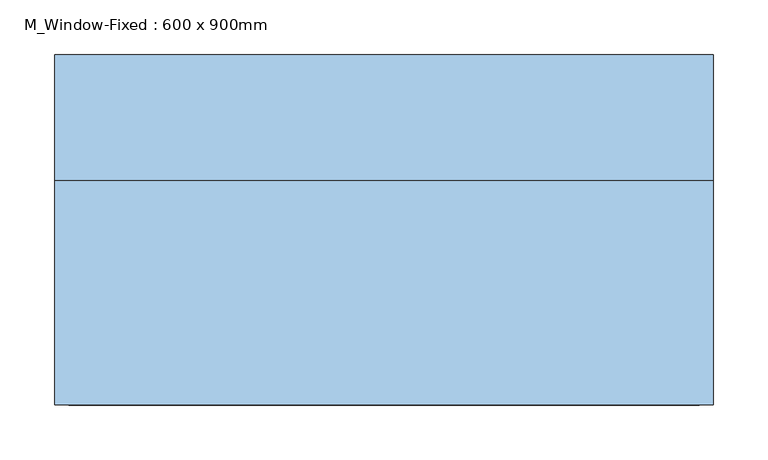
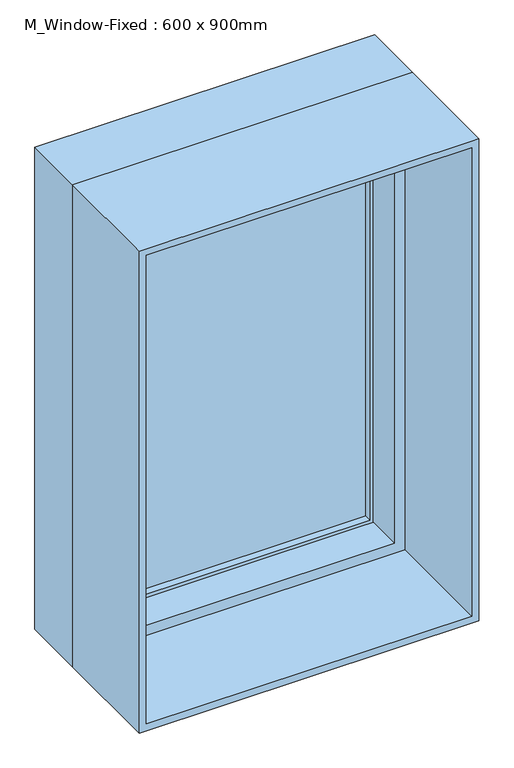
"""IFC4 building model written with IfcOpenShell, lengths in millimetres: window geometry, M_Window-Fixed : 600 x 900mm."""

import ifcopenshell
import ifcopenshell.guid

model = None  # the IFC model being written
_history = None  # IfcOwnerHistory: only IFC2X3 demands one
_inside = {}  # id of a spatial element -> (the spatial element, [elements in it])
_under = {}  # id of a project, library or spatial element -> (it, [spatial elements below it])
_declared = {}  # id of a project -> (the project, [libraries it declares])
_typed = {}  # id of a type object -> (the type object, [elements of that type])
_made_of = {}  # id of a material, layer set ... -> (it, [elements and type objects made of it])


def new_model(schema):
    """Start an empty IFC model of exactly this schema.

    Asked for "IFC4X3", IfcOpenShell would pick the latest addendum, in which some entities
    have other attributes; the version numbers below select the first issue.
    IFC2X3 requires an IfcOwnerHistory on every rooted entity: one is made here for all.
    """
    global model, _history
    if schema == "IFC4X3":
        model = ifcopenshell.file(schema_version=(4, 3, 0, 0))
    else:
        model = ifcopenshell.file(schema=schema)
    _inside.clear()
    _under.clear()
    _declared.clear()
    _typed.clear()
    _made_of.clear()
    _history = None
    if model.schema == "IFC2X3":
        org = make("IfcOrganization", Name="unknown")
        user = make(
            "IfcPersonAndOrganization",
            ThePerson=make("IfcPerson", FamilyName="unknown"),
            TheOrganization=org,
        )
        app = make(
            "IfcApplication",
            ApplicationDeveloper=org,
            Version="unknown",
            ApplicationFullName="unknown",
            ApplicationIdentifier="unknown",
        )
        _history = make(
            "IfcOwnerHistory",
            OwningUser=user,
            OwningApplication=app,
            ChangeAction="ADDED",
            CreationDate=0,
        )
    return model


def make(cls, **values):
    """One entity of the class cls with the attributes given. An attribute that is None is left unset."""
    return model.create_entity(
        cls, **{name: value for name, value in values.items() if value is not None}
    )


def rooted(cls, **values):
    """An entity with a GlobalId (a new one), such as an element, a storey or a relation."""
    return make(cls, GlobalId=ifcopenshell.guid.new(), OwnerHistory=_history, **values)


def si_unit(unit_type, name, prefix=None):
    """IfcSIUnit, for example si_unit("LENGTHUNIT", "METRE", prefix="MILLI")."""
    return make("IfcSIUnit", UnitType=unit_type, Prefix=prefix, Name=name)


def assignment(units):
    """IfcUnitAssignment: the units of a project."""
    return None if units is None else make("IfcUnitAssignment", Units=units)


def point(xyz):
    """IfcCartesianPoint."""
    return None if xyz is None else make("IfcCartesianPoint", Coordinates=xyz)


def direction(xyz):
    """IfcDirection."""
    return None if xyz is None else make("IfcDirection", DirectionRatios=xyz)


def frame(location, z_axis=None, x_axis=None):
    """IfcAxis2Placement3D, a coordinate frame: its origin and axes. An axis left out is left unset."""
    return make(
        "IfcAxis2Placement3D",
        Location=point(location),
        Axis=direction(z_axis),
        RefDirection=direction(x_axis),
    )


def origin():
    """The frame at (0, 0, 0) with its axes left unset."""
    return frame((0.0, 0.0, 0.0))


def place(relative_to, where):
    """IfcLocalPlacement: puts the frame where relative to a parent placement (None: the world)."""
    return make(
        "IfcLocalPlacement", PlacementRelTo=relative_to, RelativePlacement=where
    )


def context(
    kind, dimensions, precision=None, world=None, true_north=None, identifier=None
):
    """IfcGeometricRepresentationContext, for example the 3D "Model" context."""
    return make(
        "IfcGeometricRepresentationContext",
        ContextIdentifier=identifier,
        ContextType=kind,
        CoordinateSpaceDimension=dimensions,
        Precision=precision,
        WorldCoordinateSystem=world,
        TrueNorth=true_north,
    )


def project(units=None, contexts=None):
    """IfcProject with its units and contexts."""
    return rooted(
        "IfcProject",
        Name="project",
        RepresentationContexts=contexts,
        UnitsInContext=assignment(units),
    )


def spatial(cls, under=None, at=None, **own):
    """A site, building, storey or space (cls), placed at a placement, below another one or the project."""
    s = rooted(cls, ObjectPlacement=at, **own)
    if under is not None:
        _under.setdefault(under.id(), (under, []))[1].append(s)
    return s


def polyline(points):
    """IfcPolyline through the points."""
    return make("IfcPolyline", Points=[point(p) for p in points])


def outline(outer, holes=None, kind="AREA"):
    """IfcArbitraryClosedProfileDef: a profile drawn as a closed curve; with holes, ...WithVoids."""
    if holes is None:
        return make("IfcArbitraryClosedProfileDef", ProfileType=kind, OuterCurve=outer)
    return make(
        "IfcArbitraryProfileDefWithVoids",
        ProfileType=kind,
        OuterCurve=outer,
        InnerCurves=holes,
    )


def extrude(swept, where, along, depth):
    """IfcExtrudedAreaSolid: the profile swept, set in the frame where, extruded along a direction by depth."""
    return make(
        "IfcExtrudedAreaSolid",
        SweptArea=swept,
        Position=where,
        ExtrudedDirection=direction(along),
        Depth=depth,
    )


def faces_of(points, faces, orient=None, outer=None):
    """IfcFace entities. A face is a list of loops; a loop is a list of indices into points, from 0.

    orient and outer hold one flag for each loop. By default every Orientation is true, the
    first loop of a face is its IfcFaceOuterBound and the others are IfcFaceBound.
    """
    made = []
    for i, loops in enumerate(faces):
        bounds = []
        for j, loop in enumerate(loops):
            is_outer = j == 0 if outer is None else outer[i][j]
            bounds.append(
                make(
                    "IfcFaceOuterBound" if is_outer else "IfcFaceBound",
                    Bound=make("IfcPolyLoop", Polygon=[points[k] for k in loop]),
                    Orientation=True if orient is None else orient[i][j],
                )
            )
        made.append(make("IfcFace", Bounds=bounds))
    return made


def faceted_brep(points, faces, orient=None, outer=None, voids=None):
    """IfcFacetedBrep: a solid bounded by flat faces; with voids (closed shells), ...WithVoids."""
    shared = [point(p) for p in points]
    hull = make("IfcClosedShell", CfsFaces=faces_of(shared, faces, orient, outer))
    if voids is None:
        return make("IfcFacetedBrep", Outer=hull)
    return make(
        "IfcFacetedBrepWithVoids",
        Outer=hull,
        Voids=[
            make(cls, CfsFaces=faces_of(shared, fs, o, b)) for cls, fs, o, b in voids
        ],
    )


def shape(context_of_items, identifier, shape_type, items):
    """IfcShapeRepresentation: the items that make up one representation, for example the "Body"."""
    return make(
        "IfcShapeRepresentation",
        ContextOfItems=context_of_items,
        RepresentationIdentifier=identifier,
        RepresentationType=shape_type,
        Items=items,
    )


def source(mapping_origin, context_of_items, identifier, shape_type, items):
    """IfcRepresentationMap: a shape defined once, which mapped items show again and again."""
    return make(
        "IfcRepresentationMap",
        MappingOrigin=mapping_origin,
        MappedRepresentation=shape(context_of_items, identifier, shape_type, items),
    )


def transform(
    local_origin,
    x_axis=None,
    y_axis=None,
    z_axis=None,
    scale=None,
    scale2=None,
    scale3=None,
    uniform=True,
):
    """IfcCartesianTransformationOperator3D, or its non-uniform kind. x_axis, y_axis, z_axis: its Axis1, 2, 3."""
    if uniform:
        return make(
            "IfcCartesianTransformationOperator3D",
            Axis1=direction(x_axis),
            Axis2=direction(y_axis),
            LocalOrigin=point(local_origin),
            Scale=scale,
            Axis3=direction(z_axis),
        )
    return make(
        "IfcCartesianTransformationOperator3DnonUniform",
        Axis1=direction(x_axis),
        Axis2=direction(y_axis),
        LocalOrigin=point(local_origin),
        Scale=scale,
        Axis3=direction(z_axis),
        Scale2=scale2,
        Scale3=scale3,
    )


def mapped(mapping_source, mapping_target):
    """IfcMappedItem: shows the shape of a source again, moved by a transform."""
    return make(
        "IfcMappedItem", MappingSource=mapping_source, MappingTarget=mapping_target
    )


def made_of(thing, what):
    """Note that an element or type object is made of a material, layer set ...; save() writes the relation."""
    if what is not None:
        _made_of.setdefault(what.id(), (what, []))[1].append(thing)
    return thing


def element(
    cls,
    number,
    at=None,
    inside=None,
    cuts=None,
    type_object=None,
    material=None,
    context=None,
    identifier="Body",
    shape_type=None,
    held_by="IfcProductDefinitionShape",
    body=None,
    shapes=None,
    **own,
):
    """One element of the class cls, such as IfcWall. Its Tag is "e" and its number.

    at: its placement. inside: the storey or other place that contains it. cuts: it is an
    opening in that element (IfcRelVoidsElement). A single representation is given by context,
    identifier, shape_type and body (its items); several are given by shapes. held_by: the class
    of the entity that holds the representations. save() writes the other relations.
    """
    e = rooted(cls, Tag="e%d" % number, ObjectPlacement=at, **own)
    if body is not None:
        shapes = [shape(context, identifier, shape_type, body)]
    if shapes is not None:
        e.Representation = make(held_by, Representations=shapes)
    if inside is not None:
        _inside.setdefault(inside.id(), (inside, []))[1].append(e)
    if cuts is not None:
        rooted(
            "IfcRelVoidsElement", RelatingBuildingElement=cuts, RelatedOpeningElement=e
        )
    if type_object is not None:
        _typed.setdefault(type_object.id(), (type_object, []))[1].append(e)
    return made_of(e, material)


def aggregate(whole, parts):
    """IfcRelAggregates: a whole, such as a stair, and the parts it consists of."""
    return rooted("IfcRelAggregates", RelatingObject=whole, RelatedObjects=parts)


def save(model, path):
    """Write the relations noted so far, then the file.

    IfcRelAggregates (storeys below a building ...), IfcRelContainedInSpatialStructure (elements
    in a storey), IfcRelDefinesByType, IfcRelAssociatesMaterial and IfcRelDeclares: one each for
    every whole, place, type object, material and project.
    """
    for whole, parts in _under.values():
        aggregate(whole, parts)
    for where, things in _inside.values():
        rooted(
            "IfcRelContainedInSpatialStructure",
            RelatedElements=things,
            RelatingStructure=where,
        )
    for kind, things in _typed.values():
        rooted("IfcRelDefinesByType", RelatedObjects=things, RelatingType=kind)
    for what, things in _made_of.values():
        rooted("IfcRelAssociatesMaterial", RelatedObjects=things, RelatingMaterial=what)
    for by, libraries in _declared.values():
        rooted("IfcRelDeclares", RelatingContext=by, RelatedDefinitions=libraries)
    model.write(path)


def m_window_fixed_600_x_900mm_140d34e2(model_context):
    return source(origin(), model_context, "Body", "SolidModel", [
        faceted_brep([(300.0, 54.75, 1800.0), (300.0, 169.05, 1800.0), (-300.0, 169.05, 1800.0), (-300.0, 54.75, 1800.0), (-300.0, 169.05, 900.0), (-300.0, 54.75, 900.0), (300.0, 169.05, 900.0), (300.0, 54.75, 900.0), (268.25, 54.75, 1768.25), (268.25, 54.75, 931.75), (-268.25, 54.75, 931.75), (-268.25, 54.75, 1768.25), (-287.3, 169.05, 1787.3), (-287.3, 169.05, 912.7), (287.3, 169.05, 912.7), (287.3, 169.05, 1787.3), (268.25, 118.25, 1768.25), (-268.25, 118.25, 1768.25), (287.3, 118.25, 1787.3), (-287.3, 118.25, 1787.3), (-268.25, 118.25, 931.75), (-287.3, 118.25, 912.7), (268.25, 118.25, 931.75), (287.3, 118.25, 912.7)], [[[0, 1, 2, 3]], [[3, 2, 4, 5]], [[5, 4, 6, 7]], [[3, 5, 7, 0], [8, 9, 10, 11]], [[7, 6, 1, 0]], [[1, 6, 4, 2], [12, 13, 14, 15]], [[16, 8, 11, 17]], [[15, 18, 19, 12]], [[17, 11, 10, 20]], [[12, 19, 21, 13]], [[20, 10, 9, 22]], [[13, 21, 23, 14]], [[22, 9, 8, 16]], [[18, 23, 21, 19], [17, 20, 22, 16]], [[14, 23, 18, 15]]]),
        extrude(outline(polyline([(1800.0, -300.0), (900.0, -300.0), (900.0, 300.0), (1800.0, 300.0), (1800.0, -300.0)]), holes=[polyline([(1787.3, 287.3), (912.7, 287.3), (912.7, -287.3), (1787.3, -287.3), (1787.3, 287.3)])]), frame((0.0, -150.0, 0.0), z_axis=(0.0, 1.0, 0.0), x_axis=(0.0, 0.0, 1.0)), (0.0, 0.0, 1.0), 204.75),
        extrude(outline(polyline([(912.7, 287.3), (1787.3, 287.3), (1787.3, -287.3), (912.7, -287.3), (912.7, 287.3)]), holes=[polyline([(938.1, -261.9), (1761.9, -261.9), (1761.9, 261.9), (938.1, 261.9), (938.1, -261.9)])]), frame((0.0, 118.25, 0.0), z_axis=(0.0, 1.0, 0.0), x_axis=(0.0, 0.0, 1.0)), (0.0, 0.0, 1.0), 44.45),
        extrude(outline(polyline([(261.9, 150.0), (261.9, 143.65), (-261.9, 143.65), (-261.9, 150.0), (261.9, 150.0)])), frame((0.0, 0.0, 938.1), z_axis=(0.0, 0.0, 1.0), x_axis=(1.0, 0.0, 0.0)), (0.0, 0.0, 1.0), 823.8),
        extrude(outline(polyline([(-261.9, 130.95), (-261.9, 137.3), (261.9, 137.3), (261.9, 130.95), (-261.9, 130.95)])), frame((0.0, 0.0, 938.1), z_axis=(0.0, 0.0, 1.0), x_axis=(1.0, 0.0, 0.0)), (0.0, 0.0, 1.0), 823.8),
    ])


if __name__ == "__main__":
    model = new_model("IFC4")
    model_context = context("Model", 3, world=origin())
    ifc_project = project(units=[si_unit("LENGTHUNIT", "METRE", prefix="MILLI")], contexts=[model_context])
    site = spatial("IfcSite", under=ifc_project)
    building = spatial("IfcBuilding", under=site)
    placement = place(None, origin())
    m_window_fixed_600_x_900mm_shape = m_window_fixed_600_x_900mm_140d34e2(model_context)
    element("IfcWindow", 1, ObjectType="M_Window-Fixed : 600 x 900mm", at=placement, inside=building, context=model_context, shape_type="MappedRepresentation", body=[
        mapped(m_window_fixed_600_x_900mm_shape, transform((0.0, 0.0, 0.0), x_axis=(1.0, 0.0, 0.0), y_axis=(0.0, 1.0, 0.0), z_axis=(0.0, 0.0, 1.0))),
    ])
    save(model, "model.ifc")

# Revit data of these elements
# Type "M_Window-Fixed : 600 x 900mm"
#   Type Mark = "32"
#   Fire Rating = "0.5h"
#   Assembly Code = "B2020100"
#   Analytic Construction = "Double glazing - domestic"
#   Window Inset [instance default] = 0 cm
#   Wall Thickness [instance default] = 15 cm
#   Visual Light Transmittance = 0.81
#   Thermal Resistance (R) = 0.319569 (m²·K)/W
#   Solar Heat Gain Coefficient = 0.76
#   Rough Width = 61.5 cm
#   Rough Height = 91.5 cm
#   Interior Wall Closure [instance default] = 5.475 cm
#   Height = 90 cm
#   Heat Transfer Coefficient (U) = 3.12929 W/(m²·K)
#   Frame Extension [instance default] = 0.635 cm
#   Exterior Wall Closure [instance default] = 3.175 cm
#   Extension Jamb [instance default] = 5.475 cm
#   Default Sill Height = 90 cm
#   Width = 60 cm
#   Muntin Visibility = yes
#   Interior Trim Visibility [instance default] = yes
#   Exterior Trim Visibility [instance default] = yes
#   Extension Jamb Visibility [instance default] = yes
#   Muntin Pattern = M_Muntin Pattern_2x2 : M_Muntin Pattern_2x2
#   Interior Trim Material = Wood - Stained
#   Interior Trim = M_Trim-Window-Interior-Flat : Picture Frame
#   Interior Frame Material = Wood - Stained
#   Glass Panel Material = Glass
#   Exterior Trim Material = Clad - White
#   Exterior Trim = M_Trim-Window-Exterior-Flat : with Sill
#   Exterior Frame Material = Clad - White
#   Wall Closure = (empty or 0)
# Element 1 (IfcWindow, "M_Window-Fixed : 600 x 900mm")
#   Wall Thickness = 30 cm
#   Extension Jamb = 20.475 cm
#   Materials on its faces: "Wood - Stained", "Glass", "Clad - White"
# Materials
#   "Wood - Stained": class "Wood", colour RGB 173 132 96, transparency 0, Cost = 0
#   "Glass": class "Glass", colour RGB 245 245 243, transparency 1, Description = "Soda Lime Glass", Cost = 0
#   "Clad - White": class "Wood", colour RGB 245 245 243, transparency 0, Cost = 0
